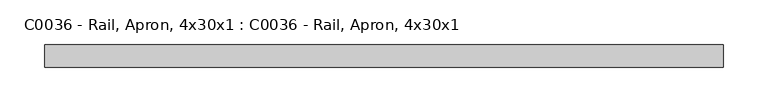
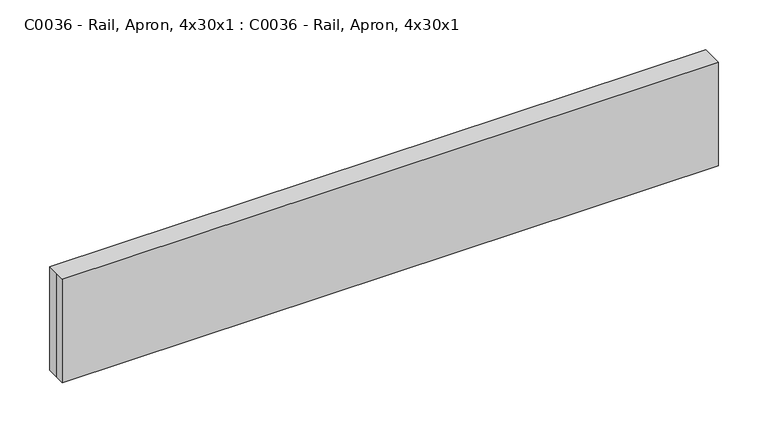
"""IFC4 building model written with IfcOpenShell, lengths in millimetres: proxy geometry, C0036 - Rail, Apron, 4x30x1 : C0036 - Rail, Apron, 4x30x1."""

import ifcopenshell
import ifcopenshell.guid

model = None  # the IFC model being written
_history = None  # IfcOwnerHistory: only IFC2X3 demands one
_inside = {}  # id of a spatial element -> (the spatial element, [elements in it])
_under = {}  # id of a project, library or spatial element -> (it, [spatial elements below it])
_declared = {}  # id of a project -> (the project, [libraries it declares])
_typed = {}  # id of a type object -> (the type object, [elements of that type])
_made_of = {}  # id of a material, layer set ... -> (it, [elements and type objects made of it])


def new_model(schema):
    """Start an empty IFC model of exactly this schema.

    Asked for "IFC4X3", IfcOpenShell would pick the latest addendum, in which some entities
    have other attributes; the version numbers below select the first issue.
    IFC2X3 requires an IfcOwnerHistory on every rooted entity: one is made here for all.
    """
    global model, _history
    if schema == "IFC4X3":
        model = ifcopenshell.file(schema_version=(4, 3, 0, 0))
    else:
        model = ifcopenshell.file(schema=schema)
    _inside.clear()
    _under.clear()
    _declared.clear()
    _typed.clear()
    _made_of.clear()
    _history = None
    if model.schema == "IFC2X3":
        org = make("IfcOrganization", Name="unknown")
        user = make(
            "IfcPersonAndOrganization",
            ThePerson=make("IfcPerson", FamilyName="unknown"),
            TheOrganization=org,
        )
        app = make(
            "IfcApplication",
            ApplicationDeveloper=org,
            Version="unknown",
            ApplicationFullName="unknown",
            ApplicationIdentifier="unknown",
        )
        _history = make(
            "IfcOwnerHistory",
            OwningUser=user,
            OwningApplication=app,
            ChangeAction="ADDED",
            CreationDate=0,
        )
    return model


def make(cls, **values):
    """One entity of the class cls with the attributes given. An attribute that is None is left unset."""
    return model.create_entity(
        cls, **{name: value for name, value in values.items() if value is not None}
    )


def rooted(cls, **values):
    """An entity with a GlobalId (a new one), such as an element, a storey or a relation."""
    return make(cls, GlobalId=ifcopenshell.guid.new(), OwnerHistory=_history, **values)


def si_unit(unit_type, name, prefix=None):
    """IfcSIUnit, for example si_unit("LENGTHUNIT", "METRE", prefix="MILLI")."""
    return make("IfcSIUnit", UnitType=unit_type, Prefix=prefix, Name=name)


def assignment(units):
    """IfcUnitAssignment: the units of a project."""
    return None if units is None else make("IfcUnitAssignment", Units=units)


def point(xyz):
    """IfcCartesianPoint."""
    return None if xyz is None else make("IfcCartesianPoint", Coordinates=xyz)


def direction(xyz):
    """IfcDirection."""
    return None if xyz is None else make("IfcDirection", DirectionRatios=xyz)


def frame(location, z_axis=None, x_axis=None):
    """IfcAxis2Placement3D, a coordinate frame: its origin and axes. An axis left out is left unset."""
    return make(
        "IfcAxis2Placement3D",
        Location=point(location),
        Axis=direction(z_axis),
        RefDirection=direction(x_axis),
    )


def origin():
    """The frame at (0, 0, 0) with its axes left unset."""
    return frame((0.0, 0.0, 0.0))


def origin_with_axes():
    """The frame at (0, 0, 0) with the z axis (0, 0, 1) and the x axis (1, 0, 0) written out."""
    return frame((0.0, 0.0, 0.0), z_axis=(0.0, 0.0, 1.0), x_axis=(1.0, 0.0, 0.0))


def place(relative_to, where):
    """IfcLocalPlacement: puts the frame where relative to a parent placement (None: the world)."""
    return make(
        "IfcLocalPlacement", PlacementRelTo=relative_to, RelativePlacement=where
    )


def context(
    kind, dimensions, precision=None, world=None, true_north=None, identifier=None
):
    """IfcGeometricRepresentationContext, for example the 3D "Model" context."""
    return make(
        "IfcGeometricRepresentationContext",
        ContextIdentifier=identifier,
        ContextType=kind,
        CoordinateSpaceDimension=dimensions,
        Precision=precision,
        WorldCoordinateSystem=world,
        TrueNorth=true_north,
    )


def project(units=None, contexts=None):
    """IfcProject with its units and contexts."""
    return rooted(
        "IfcProject",
        Name="project",
        RepresentationContexts=contexts,
        UnitsInContext=assignment(units),
    )


def spatial(cls, under=None, at=None, **own):
    """A site, building, storey or space (cls), placed at a placement, below another one or the project."""
    s = rooted(cls, ObjectPlacement=at, **own)
    if under is not None:
        _under.setdefault(under.id(), (under, []))[1].append(s)
    return s


def polyline(points):
    """IfcPolyline through the points."""
    return make("IfcPolyline", Points=[point(p) for p in points])


def outline(outer, holes=None, kind="AREA"):
    """IfcArbitraryClosedProfileDef: a profile drawn as a closed curve; with holes, ...WithVoids."""
    if holes is None:
        return make("IfcArbitraryClosedProfileDef", ProfileType=kind, OuterCurve=outer)
    return make(
        "IfcArbitraryProfileDefWithVoids",
        ProfileType=kind,
        OuterCurve=outer,
        InnerCurves=holes,
    )


def extrude(swept, where, along, depth):
    """IfcExtrudedAreaSolid: the profile swept, set in the frame where, extruded along a direction by depth."""
    return make(
        "IfcExtrudedAreaSolid",
        SweptArea=swept,
        Position=where,
        ExtrudedDirection=direction(along),
        Depth=depth,
    )


def shape(context_of_items, identifier, shape_type, items):
    """IfcShapeRepresentation: the items that make up one representation, for example the "Body"."""
    return make(
        "IfcShapeRepresentation",
        ContextOfItems=context_of_items,
        RepresentationIdentifier=identifier,
        RepresentationType=shape_type,
        Items=items,
    )


def source(mapping_origin, context_of_items, identifier, shape_type, items):
    """IfcRepresentationMap: a shape defined once, which mapped items show again and again."""
    return make(
        "IfcRepresentationMap",
        MappingOrigin=mapping_origin,
        MappedRepresentation=shape(context_of_items, identifier, shape_type, items),
    )


def transform(
    local_origin,
    x_axis=None,
    y_axis=None,
    z_axis=None,
    scale=None,
    scale2=None,
    scale3=None,
    uniform=True,
):
    """IfcCartesianTransformationOperator3D, or its non-uniform kind. x_axis, y_axis, z_axis: its Axis1, 2, 3."""
    if uniform:
        return make(
            "IfcCartesianTransformationOperator3D",
            Axis1=direction(x_axis),
            Axis2=direction(y_axis),
            LocalOrigin=point(local_origin),
            Scale=scale,
            Axis3=direction(z_axis),
        )
    return make(
        "IfcCartesianTransformationOperator3DnonUniform",
        Axis1=direction(x_axis),
        Axis2=direction(y_axis),
        LocalOrigin=point(local_origin),
        Scale=scale,
        Axis3=direction(z_axis),
        Scale2=scale2,
        Scale3=scale3,
    )


def mapped(mapping_source, mapping_target):
    """IfcMappedItem: shows the shape of a source again, moved by a transform."""
    return make(
        "IfcMappedItem", MappingSource=mapping_source, MappingTarget=mapping_target
    )


def made_of(thing, what):
    """Note that an element or type object is made of a material, layer set ...; save() writes the relation."""
    if what is not None:
        _made_of.setdefault(what.id(), (what, []))[1].append(thing)
    return thing


def element(
    cls,
    number,
    at=None,
    inside=None,
    cuts=None,
    type_object=None,
    material=None,
    context=None,
    identifier="Body",
    shape_type=None,
    held_by="IfcProductDefinitionShape",
    body=None,
    shapes=None,
    **own,
):
    """One element of the class cls, such as IfcWall. Its Tag is "e" and its number.

    at: its placement. inside: the storey or other place that contains it. cuts: it is an
    opening in that element (IfcRelVoidsElement). A single representation is given by context,
    identifier, shape_type and body (its items); several are given by shapes. held_by: the class
    of the entity that holds the representations. save() writes the other relations.
    """
    e = rooted(cls, Tag="e%d" % number, ObjectPlacement=at, **own)
    if body is not None:
        shapes = [shape(context, identifier, shape_type, body)]
    if shapes is not None:
        e.Representation = make(held_by, Representations=shapes)
    if inside is not None:
        _inside.setdefault(inside.id(), (inside, []))[1].append(e)
    if cuts is not None:
        rooted(
            "IfcRelVoidsElement", RelatingBuildingElement=cuts, RelatedOpeningElement=e
        )
    if type_object is not None:
        _typed.setdefault(type_object.id(), (type_object, []))[1].append(e)
    return made_of(e, material)


def aggregate(whole, parts):
    """IfcRelAggregates: a whole, such as a stair, and the parts it consists of."""
    return rooted("IfcRelAggregates", RelatingObject=whole, RelatedObjects=parts)


def save(model, path):
    """Write the relations noted so far, then the file.

    IfcRelAggregates (storeys below a building ...), IfcRelContainedInSpatialStructure (elements
    in a storey), IfcRelDefinesByType, IfcRelAssociatesMaterial and IfcRelDeclares: one each for
    every whole, place, type object, material and project.
    """
    for whole, parts in _under.values():
        aggregate(whole, parts)
    for where, things in _inside.values():
        rooted(
            "IfcRelContainedInSpatialStructure",
            RelatedElements=things,
            RelatingStructure=where,
        )
    for kind, things in _typed.values():
        rooted("IfcRelDefinesByType", RelatedObjects=things, RelatingType=kind)
    for what, things in _made_of.values():
        rooted("IfcRelAssociatesMaterial", RelatedObjects=things, RelatingMaterial=what)
    for by, libraries in _declared.values():
        rooted("IfcRelDeclares", RelatingContext=by, RelatedDefinitions=libraries)
    model.write(path)


def c0036_rail_apron_4x30x1_c0036_rail_apron_4x30x1_26af130f(model_context):
    return source(origin(), model_context, "Body", "SweptSolid", [
        extrude(outline(polyline([(-381.0, 12.7), (381.0, 12.7), (381.0, -12.7), (-381.0, -12.7), (-381.0, 0.0), (-381.0, 12.7)])), origin_with_axes(), (0.0, 0.0, 1.0), 127.0),
        extrude(outline(polyline([(381.0, -12.7), (-381.0, -12.7), (-381.0, 12.7), (381.0, 12.7), (381.0, -12.7)])), origin_with_axes(), (0.0, 0.0, 1.0), 127.0),
    ])


if __name__ == "__main__":
    model = new_model("IFC4")
    model_context = context("Model", 3, world=origin())
    ifc_project = project(units=[si_unit("LENGTHUNIT", "METRE", prefix="MILLI")], contexts=[model_context])
    site = spatial("IfcSite", under=ifc_project)
    building = spatial("IfcBuilding", under=site)
    placement = place(None, origin())
    c0036_rail_apron_4x30x1_c0036_rail_apron_4x30x1_shape = c0036_rail_apron_4x30x1_c0036_rail_apron_4x30x1_26af130f(model_context)
    element("IfcBuildingElementProxy", 1, Name="C0036 - Rail, Apron, 4x30x1 : C0036 - Rail, Apron, 4x30x1", ObjectType="C0036 - Rail, Apron, 4x30x1 : C0036 - Rail, Apron, 4x30x1", at=placement, inside=building, context=model_context, shape_type="MappedRepresentation", body=[
        mapped(c0036_rail_apron_4x30x1_c0036_rail_apron_4x30x1_shape, transform((0.0, 0.0, 0.0), x_axis=(1.0, 0.0, 0.0), y_axis=(0.0, 1.0, 0.0), z_axis=(0.0, 0.0, 1.0))),
    ])
    save(model, "model.ifc")

# Revit data of these elements
# Type "C0036 - Rail, Apron, 4x30x1 : C0036 - Rail, Apron, 4x30x1"
#   Watts2 = "0"
#   Watts1 = "0"
#   Unit_Issue = "EA"
#   UTIL_6_Misc = "-"
#   UTIL_5_NonMedGas = "-"
#   UTIL_4_MiscGas = "-"
#   UTIL_3_MedGas = "-"
#   UTIL_2_Elec = "-"
#   UTIL_1_WaterDrain = "-"
#   Nomenclature = "Rail, Apron, 4x30x1"
#   NSN = "6530"
#   Location [instance default] = ""
#   JSN = "C0036"
#   Fund_Source_VA = "-"
#   Fund_Source_Navy = "-"
#   Fund_Source_Army = "-"
#   Fund_Source_AF = "-"
#   ELEC_Volts2 = "0"
#   ELEC_Volts1 = "0"
#   ELEC_Phase2 = "0"
#   ELEC_Phase1 = "0"
#   ELEC_HertzSwitch = "0"
#   ELEC_HertzDependent = "0"
#   ELEC_Hertz = "0"
#   ELEC_Amps2 = "0"
#   ELEC_Amps1 = "0"
#   DetailDescription = "Apron rail. Also referred to as an apron front, apron panel, or knee space rail. Used to close in front knee space area and/or provide work surface support between two base cabinets or a base cabinet and wall. Apron rails should be ordered in pairs to provide both front and rear work surface support."
#   CAT_VA = "A"
#   CAT_Navy = "A"
#   CAT_IHS = "-"
#   CAT_Army = "A"
#   CAT_AF = "A"
#   BTUperhour = "0"
#   Weight_IP = 9
#   DIM_Width_IP = 2' - 6"
#   DIM_Height_IP = 0' - 5"
#   DIM_Depth_IP = 0' - 1"
#   Top Panel Material = none
#   Toe Panel Material = none
#   Side Panel Material = none
#   Shelf Panel Material = none
#   Drawer Front Material = none
#   Door Panel Material = none
#   Back Panel Material = none
#   Assembly Code = ""
# Element 1 (IfcBuildingElementProxy, "C0036 - Rail, Apron, 4x30x1 : C0036 - Rail, Apron, 4x30x1")
#   Materials on its faces: "EquipSpace"
# Materials
#   "EquipSpace": class "Unassigned", colour RGB 221 217 195, transparency 0.5
